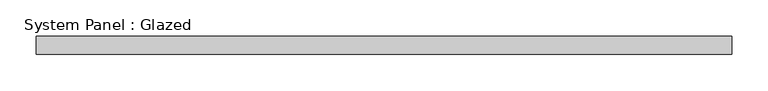
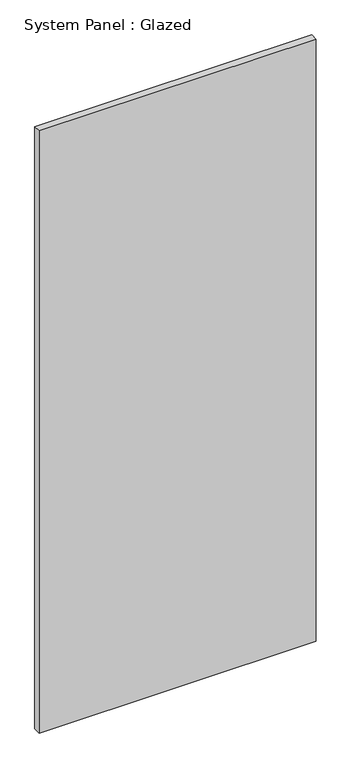
"""IFC4 building model written with IfcOpenShell, lengths in millimetres: plate geometry, System Panel : Glazed."""

from ifc_helpers import new_model, si_unit, origin, origin_with_axes, place, context, project, spatial, polyline, outline, extrude, source, transform, mapped, element, save


def system_panel_glazed_8c511674(model_context):
    return source(origin(), model_context, "Body", "SweptSolid", [
        extrude(outline(polyline([(482.5999999, -44.45), (-482.5999999, -44.45), (-482.5999999, -19.05), (482.5999999, -19.05), (482.5999999, -44.45)])), origin_with_axes(), (0.0, 0.0, 1.0), 2216.15),
    ])


if __name__ == "__main__":
    model = new_model("IFC4")
    model_context = context("Model", 3, world=origin())
    ifc_project = project(units=[si_unit("LENGTHUNIT", "METRE", prefix="MILLI")], contexts=[model_context])
    site = spatial("IfcSite", under=ifc_project)
    building = spatial("IfcBuilding", under=site)
    placement = place(None, origin())
    system_panel_glazed_shape = system_panel_glazed_8c511674(model_context)
    element("IfcPlate", 1, ObjectType="System Panel : Glazed", at=placement, inside=building, context=model_context, shape_type="MappedRepresentation", body=[
        mapped(system_panel_glazed_shape, transform((0.0, 0.0, 0.0), x_axis=(1.0, 0.0, 0.0), y_axis=(0.0, 1.0, 0.0), z_axis=(0.0, 0.0, 1.0))),
    ])
    save(model, "model.ifc")

# Revit data of these elements
# Type "System Panel : Glazed"
#   Construction Type Id = "GSP4R"
#   Analytic Construction = "1/8 in Pilkington single glazing"
#   Visual Light Transmittance = 0.9
#   Solar Heat Gain Coefficient = 0.86
#   Heat Transfer Coefficient (U) = 1.18115 BTU/(h·ft²·°F)
#   Define Thermal Properties by = 1
# Element 1 (IfcPlate, "System Panel : Glazed")
#   Materials on its faces: "Glass"
# Materials
#   "Glass": class "Glass", colour RGB 0 128 192, transparency 0.75, Description = "Soda Lime Glass", Cost = 0
